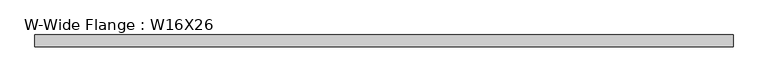
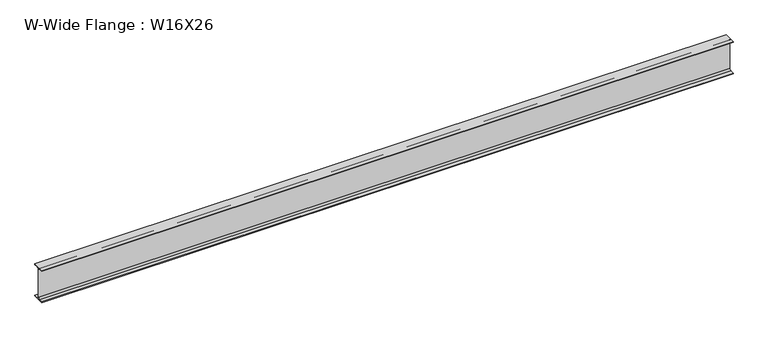
"""IFC4 building model written with IfcOpenShell, lengths in millimetres: beam geometry, W-Wide Flange : W16X26."""

from ifc_helpers import new_model, si_unit, point, frame, frame_2d, origin, place, context, project, spatial, polyline, circle_curve, trimmed, segment, composite_curve, outline, extrude, source, transform, mapped, element, save


def w_wide_flange_w16x26_3658d20b(model_context):
    return source(origin(), model_context, "Body", "SweptSolid", [
        extrude(outline(composite_curve([segment(polyline([(69.85, -190.627), (69.85, -199.39), (-69.85, -199.39), (-69.85, -190.627), (-21.3995, -190.627)]), True, "CONTINUOUS"), segment(trimmed(circle_curve(frame_2d((-21.3995, -172.4025)), 18.2245), [point((-21.3995, -190.627))], [point((-3.175, -172.4025))], True, "CARTESIAN"), True, "CONTINUOUS"), segment(polyline([(-3.175, -172.4025), (-3.175, 172.4025)]), True, "CONTINUOUS"), segment(trimmed(circle_curve(frame_2d((-21.3995, 172.4025)), 18.2245), [point((-3.175, 172.4025))], [point((-21.3995, 190.627))], True, "CARTESIAN"), True, "CONTINUOUS"), segment(polyline([(-21.3995, 190.627), (-69.85, 190.627), (-69.85, 199.39), (69.85, 199.39), (69.85, 190.627), (21.3995, 190.627)]), True, "CONTINUOUS"), segment(trimmed(circle_curve(frame_2d((21.3995, 172.4025)), 18.2245), [point((21.3995, 190.627))], [point((3.175, 172.4025))], True, "CARTESIAN"), True, "CONTINUOUS"), segment(polyline([(3.175, 172.4025), (3.175, -172.4025)]), True, "CONTINUOUS"), segment(trimmed(circle_curve(frame_2d((21.3995, -172.4025)), 18.2245), [point((3.175, -172.4025))], [point((21.3995, -190.627))], True, "CARTESIAN"), True, "CONTINUOUS"), segment(polyline([(21.3995, -190.627), (69.85, -190.627)]), True, "CONTINUOUS")], self_intersect=False)), frame((-4105.2253906, 0.0, 0.0), z_axis=(1.0, 0.0, 0.0), x_axis=(0.0, 1.0, 0.0)), (0.0, 0.0, 1.0), 8138.2195313),
    ])


if __name__ == "__main__":
    model = new_model("IFC4")
    model_context = context("Model", 3, world=origin())
    ifc_project = project(units=[si_unit("LENGTHUNIT", "METRE", prefix="MILLI")], contexts=[model_context])
    site = spatial("IfcSite", under=ifc_project)
    building = spatial("IfcBuilding", under=site)
    placement = place(None, origin())
    w_wide_flange_w16x26_shape = w_wide_flange_w16x26_3658d20b(model_context)
    element("IfcBeam", 1, ObjectType="W-Wide Flange : W16X26", at=placement, inside=building, context=model_context, shape_type="MappedRepresentation", body=[
        mapped(w_wide_flange_w16x26_shape, transform((0.0, 0.0, 0.0), x_axis=(1.0, 0.0, 0.0), y_axis=(0.0, 1.0, 0.0), z_axis=(0.0, 0.0, 1.0))),
    ])
    save(model, "model.ifc")

# Revit data of these elements
# Type "W-Wide Flange : W16X26"
#   Assembly Code = "B10"
#   W = 26
#   Length [instance default] = 1524 mm
#   bf = 139.7 mm
#   d = 398.78 mm
#   k = 26.988 mm
#   k2 = 18.225 mm
#   tf = 8.763 mm
#   tw = 6.35 mm
#   A = 0.00495483 m²
#   Structural Material [instance default] = Steel ASTM A992
# Element 1 (IfcBeam, "W-Wide Flange : W16X26")
#   Structural Material = Aluminum, Anodized Red
#   Materials on its faces: "Aluminum, Anodized Red"
# Materials
#   "Steel ASTM A992": class "Metal", colour RGB 128 0 0, transparency 0, Description = "Structural steel 50ksi", Cost = 0
#   "Aluminum, Anodized Red": class "Metal", colour RGB 120 120 120, transparency 0, Description = "Anodized aluminum, red", Cost = 0
